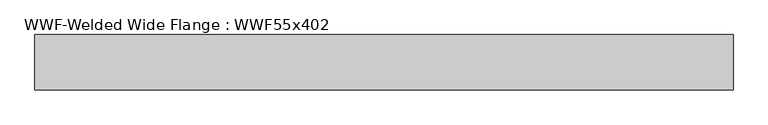
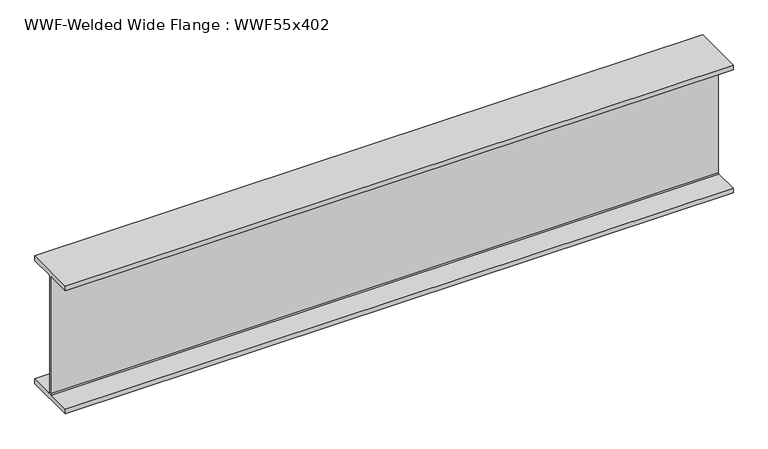
"""IFC4 building model written with IfcOpenShell, lengths in millimetres: beam geometry, WWF-Welded Wide Flange : WWF55x402."""

import ifcopenshell
import ifcopenshell.guid

model = None  # the IFC model being written
_history = None  # IfcOwnerHistory: only IFC2X3 demands one
_inside = {}  # id of a spatial element -> (the spatial element, [elements in it])
_under = {}  # id of a project, library or spatial element -> (it, [spatial elements below it])
_declared = {}  # id of a project -> (the project, [libraries it declares])
_typed = {}  # id of a type object -> (the type object, [elements of that type])
_made_of = {}  # id of a material, layer set ... -> (it, [elements and type objects made of it])


def new_model(schema):
    """Start an empty IFC model of exactly this schema.

    Asked for "IFC4X3", IfcOpenShell would pick the latest addendum, in which some entities
    have other attributes; the version numbers below select the first issue.
    IFC2X3 requires an IfcOwnerHistory on every rooted entity: one is made here for all.
    """
    global model, _history
    if schema == "IFC4X3":
        model = ifcopenshell.file(schema_version=(4, 3, 0, 0))
    else:
        model = ifcopenshell.file(schema=schema)
    _inside.clear()
    _under.clear()
    _declared.clear()
    _typed.clear()
    _made_of.clear()
    _history = None
    if model.schema == "IFC2X3":
        org = make("IfcOrganization", Name="unknown")
        user = make(
            "IfcPersonAndOrganization",
            ThePerson=make("IfcPerson", FamilyName="unknown"),
            TheOrganization=org,
        )
        app = make(
            "IfcApplication",
            ApplicationDeveloper=org,
            Version="unknown",
            ApplicationFullName="unknown",
            ApplicationIdentifier="unknown",
        )
        _history = make(
            "IfcOwnerHistory",
            OwningUser=user,
            OwningApplication=app,
            ChangeAction="ADDED",
            CreationDate=0,
        )
    return model


def make(cls, **values):
    """One entity of the class cls with the attributes given. An attribute that is None is left unset."""
    return model.create_entity(
        cls, **{name: value for name, value in values.items() if value is not None}
    )


def rooted(cls, **values):
    """An entity with a GlobalId (a new one), such as an element, a storey or a relation."""
    return make(cls, GlobalId=ifcopenshell.guid.new(), OwnerHistory=_history, **values)


def si_unit(unit_type, name, prefix=None):
    """IfcSIUnit, for example si_unit("LENGTHUNIT", "METRE", prefix="MILLI")."""
    return make("IfcSIUnit", UnitType=unit_type, Prefix=prefix, Name=name)


def assignment(units):
    """IfcUnitAssignment: the units of a project."""
    return None if units is None else make("IfcUnitAssignment", Units=units)


def point(xyz):
    """IfcCartesianPoint."""
    return None if xyz is None else make("IfcCartesianPoint", Coordinates=xyz)


def direction(xyz):
    """IfcDirection."""
    return None if xyz is None else make("IfcDirection", DirectionRatios=xyz)


def frame(location, z_axis=None, x_axis=None):
    """IfcAxis2Placement3D, a coordinate frame: its origin and axes. An axis left out is left unset."""
    return make(
        "IfcAxis2Placement3D",
        Location=point(location),
        Axis=direction(z_axis),
        RefDirection=direction(x_axis),
    )


def origin():
    """The frame at (0, 0, 0) with its axes left unset."""
    return frame((0.0, 0.0, 0.0))


def place(relative_to, where):
    """IfcLocalPlacement: puts the frame where relative to a parent placement (None: the world)."""
    return make(
        "IfcLocalPlacement", PlacementRelTo=relative_to, RelativePlacement=where
    )


def context(
    kind, dimensions, precision=None, world=None, true_north=None, identifier=None
):
    """IfcGeometricRepresentationContext, for example the 3D "Model" context."""
    return make(
        "IfcGeometricRepresentationContext",
        ContextIdentifier=identifier,
        ContextType=kind,
        CoordinateSpaceDimension=dimensions,
        Precision=precision,
        WorldCoordinateSystem=world,
        TrueNorth=true_north,
    )


def project(units=None, contexts=None):
    """IfcProject with its units and contexts."""
    return rooted(
        "IfcProject",
        Name="project",
        RepresentationContexts=contexts,
        UnitsInContext=assignment(units),
    )


def spatial(cls, under=None, at=None, **own):
    """A site, building, storey or space (cls), placed at a placement, below another one or the project."""
    s = rooted(cls, ObjectPlacement=at, **own)
    if under is not None:
        _under.setdefault(under.id(), (under, []))[1].append(s)
    return s


def polyline(points):
    """IfcPolyline through the points."""
    return make("IfcPolyline", Points=[point(p) for p in points])


def outline(outer, holes=None, kind="AREA"):
    """IfcArbitraryClosedProfileDef: a profile drawn as a closed curve; with holes, ...WithVoids."""
    if holes is None:
        return make("IfcArbitraryClosedProfileDef", ProfileType=kind, OuterCurve=outer)
    return make(
        "IfcArbitraryProfileDefWithVoids",
        ProfileType=kind,
        OuterCurve=outer,
        InnerCurves=holes,
    )


def extrude(swept, where, along, depth):
    """IfcExtrudedAreaSolid: the profile swept, set in the frame where, extruded along a direction by depth."""
    return make(
        "IfcExtrudedAreaSolid",
        SweptArea=swept,
        Position=where,
        ExtrudedDirection=direction(along),
        Depth=depth,
    )


def shape(context_of_items, identifier, shape_type, items):
    """IfcShapeRepresentation: the items that make up one representation, for example the "Body"."""
    return make(
        "IfcShapeRepresentation",
        ContextOfItems=context_of_items,
        RepresentationIdentifier=identifier,
        RepresentationType=shape_type,
        Items=items,
    )


def source(mapping_origin, context_of_items, identifier, shape_type, items):
    """IfcRepresentationMap: a shape defined once, which mapped items show again and again."""
    return make(
        "IfcRepresentationMap",
        MappingOrigin=mapping_origin,
        MappedRepresentation=shape(context_of_items, identifier, shape_type, items),
    )


def transform(
    local_origin,
    x_axis=None,
    y_axis=None,
    z_axis=None,
    scale=None,
    scale2=None,
    scale3=None,
    uniform=True,
):
    """IfcCartesianTransformationOperator3D, or its non-uniform kind. x_axis, y_axis, z_axis: its Axis1, 2, 3."""
    if uniform:
        return make(
            "IfcCartesianTransformationOperator3D",
            Axis1=direction(x_axis),
            Axis2=direction(y_axis),
            LocalOrigin=point(local_origin),
            Scale=scale,
            Axis3=direction(z_axis),
        )
    return make(
        "IfcCartesianTransformationOperator3DnonUniform",
        Axis1=direction(x_axis),
        Axis2=direction(y_axis),
        LocalOrigin=point(local_origin),
        Scale=scale,
        Axis3=direction(z_axis),
        Scale2=scale2,
        Scale3=scale3,
    )


def mapped(mapping_source, mapping_target):
    """IfcMappedItem: shows the shape of a source again, moved by a transform."""
    return make(
        "IfcMappedItem", MappingSource=mapping_source, MappingTarget=mapping_target
    )


def made_of(thing, what):
    """Note that an element or type object is made of a material, layer set ...; save() writes the relation."""
    if what is not None:
        _made_of.setdefault(what.id(), (what, []))[1].append(thing)
    return thing


def element(
    cls,
    number,
    at=None,
    inside=None,
    cuts=None,
    type_object=None,
    material=None,
    context=None,
    identifier="Body",
    shape_type=None,
    held_by="IfcProductDefinitionShape",
    body=None,
    shapes=None,
    **own,
):
    """One element of the class cls, such as IfcWall. Its Tag is "e" and its number.

    at: its placement. inside: the storey or other place that contains it. cuts: it is an
    opening in that element (IfcRelVoidsElement). A single representation is given by context,
    identifier, shape_type and body (its items); several are given by shapes. held_by: the class
    of the entity that holds the representations. save() writes the other relations.
    """
    e = rooted(cls, Tag="e%d" % number, ObjectPlacement=at, **own)
    if body is not None:
        shapes = [shape(context, identifier, shape_type, body)]
    if shapes is not None:
        e.Representation = make(held_by, Representations=shapes)
    if inside is not None:
        _inside.setdefault(inside.id(), (inside, []))[1].append(e)
    if cuts is not None:
        rooted(
            "IfcRelVoidsElement", RelatingBuildingElement=cuts, RelatedOpeningElement=e
        )
    if type_object is not None:
        _typed.setdefault(type_object.id(), (type_object, []))[1].append(e)
    return made_of(e, material)


def aggregate(whole, parts):
    """IfcRelAggregates: a whole, such as a stair, and the parts it consists of."""
    return rooted("IfcRelAggregates", RelatingObject=whole, RelatedObjects=parts)


def save(model, path):
    """Write the relations noted so far, then the file.

    IfcRelAggregates (storeys below a building ...), IfcRelContainedInSpatialStructure (elements
    in a storey), IfcRelDefinesByType, IfcRelAssociatesMaterial and IfcRelDeclares: one each for
    every whole, place, type object, material and project.
    """
    for whole, parts in _under.values():
        aggregate(whole, parts)
    for where, things in _inside.values():
        rooted(
            "IfcRelContainedInSpatialStructure",
            RelatedElements=things,
            RelatingStructure=where,
        )
    for kind, things in _typed.values():
        rooted("IfcRelDefinesByType", RelatedObjects=things, RelatingType=kind)
    for what, things in _made_of.values():
        rooted("IfcRelAssociatesMaterial", RelatedObjects=things, RelatingMaterial=what)
    for by, libraries in _declared.values():
        rooted("IfcRelDeclares", RelatingContext=by, RelatedDefinitions=libraries)
    model.write(path)


def wwf_welded_wide_flange_wwf55x402_e70519e9(model_context):
    return source(origin(), model_context, "Body", "SweptSolid", [
        extrude(outline(polyline([(274.955, -649.986), (274.955, -700.024), (-274.955, -700.024), (-274.955, -649.986), (-19.05, -649.986), (-8.001, -638.937), (-8.001, 638.937), (-19.05, 649.986), (-274.955, 649.986), (-274.955, 700.024), (274.955, 700.024), (274.955, 649.986), (19.05, 649.986), (8.001, 638.937), (8.001, -638.937), (19.05, -649.986), (274.955, -649.986)])), frame((-3459.5195507, 0.0, 0.0), z_axis=(1.0, 0.0, 0.0), x_axis=(0.0, 1.0, 0.0)), (0.0, 0.0, 1.0), 6931.739102),
    ])


if __name__ == "__main__":
    model = new_model("IFC4")
    model_context = context("Model", 3, world=origin())
    ifc_project = project(units=[si_unit("LENGTHUNIT", "METRE", prefix="MILLI")], contexts=[model_context])
    site = spatial("IfcSite", under=ifc_project)
    building = spatial("IfcBuilding", under=site)
    placement = place(None, origin())
    wwf_welded_wide_flange_wwf55x402_shape = wwf_welded_wide_flange_wwf55x402_e70519e9(model_context)
    element("IfcBeam", 1, ObjectType="WWF-Welded Wide Flange : WWF55x402", at=placement, inside=building, context=model_context, shape_type="MappedRepresentation", body=[
        mapped(wwf_welded_wide_flange_wwf55x402_shape, transform((0.0, 0.0, 0.0), x_axis=(1.0, 0.0, 0.0), y_axis=(0.0, 1.0, 0.0), z_axis=(0.0, 0.0, 1.0))),
    ])
    save(model, "model.ifc")

# Revit data of these elements
# Type "WWF-Welded Wide Flange : WWF55x402"
#   Assembly Code = "B10"
#   Nominal d = "12"
#   W = 402
#   Length [instance default] = 1524 mm
#   bf = 549.91 mm
#   d = 1400.048 mm
#   k = 19.05 mm
#   tf = 50.038 mm
#   tw = 16.002 mm
#   A = 0.0761289 m²
#   Structural Material [instance default] = Steel ASTM A572
# Element 1 (IfcBeam, "WWF-Welded Wide Flange : WWF55x402")
#   Structural Material = Metal - Steel 43-275
#   Materials on its faces: "Metal - Steel 43-275"
# Materials
#   "Steel ASTM A572": class "Metal", colour RGB 247 247 247, transparency 0, Description = "Structural steel, high strength low alloy, ASTM - A572 - 50", Cost = 0
#   "Metal - Steel 43-275": class "Metal", colour RGB 247 247 247, transparency 0, Cost = 0
